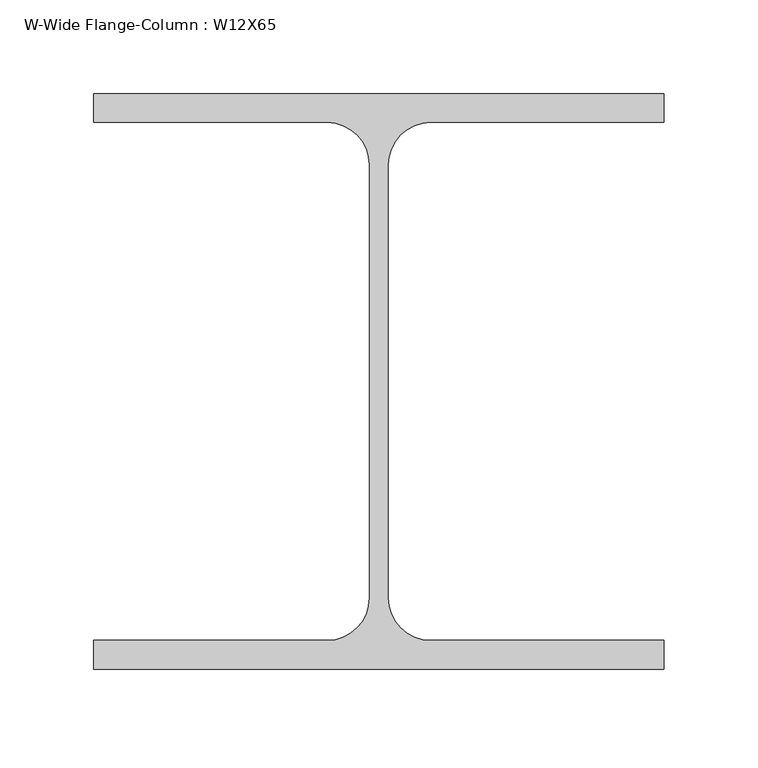
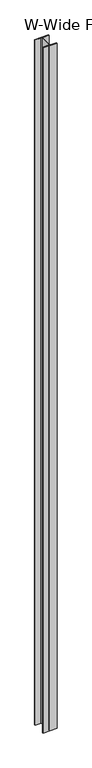
"""IFC4 building model written with IfcOpenShell, lengths in millimetres: column geometry, W-Wide Flange-Column : W12X65."""

from ifc_helpers import new_model, si_unit, point, frame, frame_2d, origin, place, context, project, spatial, polyline, circle_curve, trimmed, segment, composite_curve, outline, extrude, source, transform, mapped, element, save


def w_wide_flange_column_w12x65_0830fbe6(model_context):
    return source(origin(), model_context, "Body", "SweptSolid", [
        extrude(outline(composite_curve([segment(polyline([(152.4, 153.67), (152.4, 138.303), (27.686, 138.303)]), True, "CONTINUOUS"), segment(trimmed(circle_curve(frame_2d((27.686, 115.57)), 22.733), [point((27.686, 138.303))], [point((4.953, 115.57))], True, "CARTESIAN"), True, "CONTINUOUS"), segment(polyline([(4.953, 115.57), (4.953, -115.57)]), True, "CONTINUOUS"), segment(trimmed(circle_curve(frame_2d((27.686, -115.57)), 22.733), [point((4.953, -115.57))], [point((27.686, -138.303))], True, "CARTESIAN"), True, "CONTINUOUS"), segment(polyline([(27.686, -138.303), (152.4, -138.303), (152.4, -153.67), (-152.4, -153.67), (-152.4, -138.303), (-27.686, -138.303)]), True, "CONTINUOUS"), segment(trimmed(circle_curve(frame_2d((-27.686, -115.57)), 22.733), [point((-27.686, -138.303))], [point((-4.953, -115.57))], True, "CARTESIAN"), True, "CONTINUOUS"), segment(polyline([(-4.953, -115.57), (-4.953, 115.57)]), True, "CONTINUOUS"), segment(trimmed(circle_curve(frame_2d((-27.686, 115.57)), 22.733), [point((-4.953, 115.57))], [point((-27.686, 138.303))], True, "CARTESIAN"), True, "CONTINUOUS"), segment(polyline([(-27.686, 138.303), (-152.4, 138.303), (-152.4, 153.67), (152.4, 153.67)]), True, "CONTINUOUS")], self_intersect=False)), frame((0.0, 0.0, 11849.1), z_axis=(0.0, 0.0, 1.0), x_axis=(1.0, 0.0, 0.0)), (0.0, 0.0, 1.0), 15735.3),
    ])


if __name__ == "__main__":
    model = new_model("IFC4")
    model_context = context("Model", 3, world=origin())
    ifc_project = project(units=[si_unit("LENGTHUNIT", "METRE", prefix="MILLI")], contexts=[model_context])
    site = spatial("IfcSite", under=ifc_project)
    building = spatial("IfcBuilding", under=site)
    placement = place(None, origin())
    w_wide_flange_column_w12x65_shape = w_wide_flange_column_w12x65_0830fbe6(model_context)
    element("IfcColumn", 1, ObjectType="W-Wide Flange-Column : W12X65", at=placement, inside=building, context=model_context, shape_type="MappedRepresentation", body=[
        mapped(w_wide_flange_column_w12x65_shape, transform((0.0, 0.0, 0.0), x_axis=(1.0, 0.0, 0.0), y_axis=(0.0, 1.0, 0.0), z_axis=(0.0, 0.0, 1.0))),
    ])
    save(model, "model.ifc")

# Revit data of these elements
# Type "W-Wide Flange-Column : W12X65"
#   Assembly Code = "B10"
#   W = 65
#   bf = 1' - 0"
#   d = 1' - 0.1"
#   k = 0' - 1 1/2"
#   kr = 0' - 0.895"
#   tf = 0' - 0.605"
#   tw = 0' - 0.39"
#   A = 0.132639 SF
#   Structural Material [instance default] = Steel ASTM A992
# Element 1 (IfcColumn, "W-Wide Flange-Column : W12X65")
#   Materials on its faces: "Steel ASTM A992"
# Materials
#   "Steel ASTM A992": class "Metal", colour RGB 199 199 199, transparency 0, Description = "Structural steel 50ksi", Cost = 0
